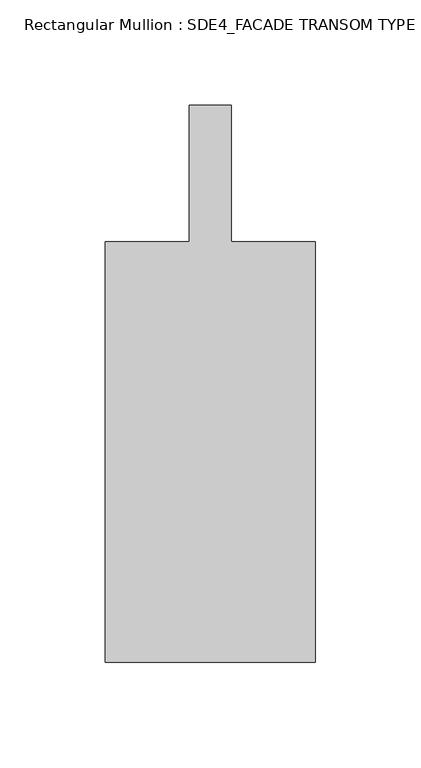
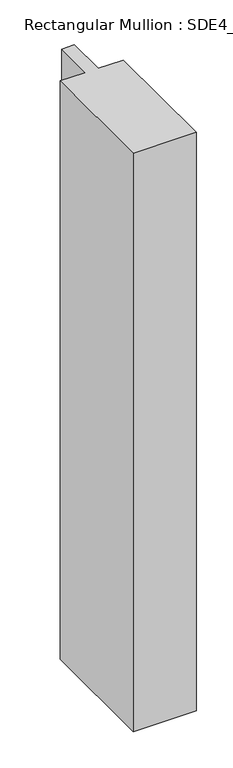
"""IFC4 building model written with IfcOpenShell, lengths in millimetres: member geometry, Rectangular Mullion : SDE4_FACADE TRANSOM TYPE 2."""

from ifc_helpers import new_model, si_unit, frame, origin, place, context, project, spatial, polyline, outline, extrude, source, transform, mapped, element, save


def rectangular_mullion_sde4_facade_transom_type_2_3dd3124f(model_context):
    return source(origin(), model_context, "Body", "SweptSolid", [
        extrude(outline(polyline([(50.0, -132.5), (-50.0, -132.5), (-50.0, 67.5), (-10.0, 67.5), (-10.0, 132.5), (10.0, 132.5), (10.0, 67.5), (50.0, 67.5), (50.0, -132.5)])), frame((0.0, 0.0, -967.5), z_axis=(0.0, 0.0, 1.0), x_axis=(1.0, 0.0, 0.0)), (0.0, 0.0, 1.0), 967.5),
    ])


if __name__ == "__main__":
    model = new_model("IFC4")
    model_context = context("Model", 3, world=origin())
    ifc_project = project(units=[si_unit("LENGTHUNIT", "METRE", prefix="MILLI")], contexts=[model_context])
    site = spatial("IfcSite", under=ifc_project)
    building = spatial("IfcBuilding", under=site)
    placement = place(None, origin())
    rectangular_mullion_sde4_facade_transom_type_2_shape = rectangular_mullion_sde4_facade_transom_type_2_3dd3124f(model_context)
    element("IfcMember", 1, ObjectType="Rectangular Mullion : SDE4_FACADE TRANSOM TYPE 2", at=placement, inside=building, context=model_context, shape_type="MappedRepresentation", body=[
        mapped(rectangular_mullion_sde4_facade_transom_type_2_shape, transform((0.0, 0.0, 0.0), x_axis=(1.0, 0.0, 0.0), y_axis=(0.0, 1.0, 0.0), z_axis=(0.0, 0.0, 1.0))),
    ])
    save(model, "model.ifc")

# Revit data of these elements
# Type "Rectangular Mullion : SDE4_FACADE TRANSOM TYPE 2"
#   built-in parameter 1007322 = 0.869423 (stored number, unit not read)
#   built-in parameter 1007321 = 0.164042 (stored number, unit not read)
#   built-in parameter 1007320 = 0.164042 (stored number, unit not read)
